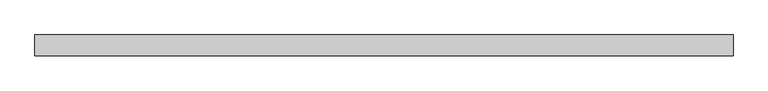
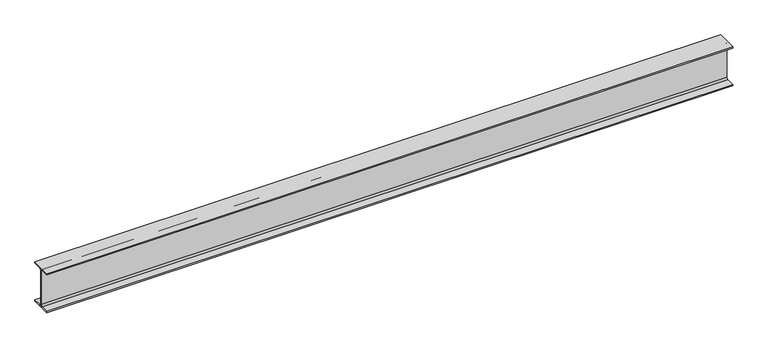
"""IFC4 building model written with IfcOpenShell, lengths in millimetres: beam geometry, 0912_Steel Framing_H-KSD3502 : H_SB_ASB_H-350x175x7x11."""

from ifc_helpers import new_model, si_unit, point, frame, frame_2d, origin, place, context, project, spatial, polyline, circle_curve, trimmed, segment, composite_curve, outline, extrude, source, transform, mapped, element, save


def beam_b532c406(model_context):
    return source(origin(), model_context, "Body", "SweptSolid", [
        extrude(outline(composite_curve([segment(polyline([(87.5, -164.0), (87.5, -175.0), (-87.5, -175.0), (-87.5, -164.0), (-17.5, -164.0)]), True, "CONTINUOUS"), segment(trimmed(circle_curve(frame_2d((-17.5, -150.0)), 14.0), [point((-17.5, -164.0))], [point((-3.5, -150.0))], True, "CARTESIAN"), True, "CONTINUOUS"), segment(polyline([(-3.5, -150.0), (-3.5, 150.0)]), True, "CONTINUOUS"), segment(trimmed(circle_curve(frame_2d((-17.5, 150.0)), 14.0), [point((-3.5, 150.0))], [point((-17.5, 164.0))], True, "CARTESIAN"), True, "CONTINUOUS"), segment(polyline([(-17.5, 164.0), (-87.5, 164.0), (-87.5, 175.0), (87.5, 175.0), (87.5, 164.0), (17.5, 164.0)]), True, "CONTINUOUS"), segment(trimmed(circle_curve(frame_2d((17.5, 150.0)), 14.0), [point((17.5, 164.0))], [point((3.5, 150.0))], True, "CARTESIAN"), True, "CONTINUOUS"), segment(polyline([(3.5, 150.0), (3.5, -150.0)]), True, "CONTINUOUS"), segment(trimmed(circle_curve(frame_2d((17.5, -150.0)), 14.0), [point((3.5, -150.0))], [point((17.5, -164.0))], True, "CARTESIAN"), True, "CONTINUOUS"), segment(polyline([(17.5, -164.0), (87.5, -164.0)]), True, "CONTINUOUS")], self_intersect=False)), frame((-2774.336211, 0.0, 0.0), z_axis=(1.0, 0.0, 0.0), x_axis=(0.0, 1.0, 0.0)), (0.0, 0.0, 1.0), 5797.2714142),
    ])


if __name__ == "__main__":
    model = new_model("IFC4")
    model_context = context("Model", 3, world=origin())
    ifc_project = project(units=[si_unit("LENGTHUNIT", "METRE", prefix="MILLI")], contexts=[model_context])
    site = spatial("IfcSite", under=ifc_project)
    building = spatial("IfcBuilding", under=site)
    placement = place(None, origin())
    beam_shape = beam_b532c406(model_context)
    element("IfcBeam", 1, ObjectType="0912_Steel Framing_H-KSD3502 : H_SB_ASB_H-350x175x7x11", at=placement, inside=building, context=model_context, shape_type="MappedRepresentation", body=[
        mapped(beam_shape, transform((0.0, 0.0, 0.0), x_axis=(1.0, 0.0, 0.0), y_axis=(0.0, 1.0, 0.0), z_axis=(0.0, 0.0, 1.0))),
    ])
    save(model, "model.ifc")

# Revit data of these elements
# Type "0912_Steel Framing_H-KSD3502 : H_SB_ASB_H-350x175x7x11"
#   H_WM Code_1 = "S01AA002-00001 | Main Steel Structure Fabrication Work | Shelter/Building | Medium Steel - Standard (90KG/M>Weight≥30KG/M) | Material: (   )"
#   H_WM Code_2 = "S03AA028-00001 | Main Steel Structure Erection Work | Shelter/Building | Medium Steel (90KG/M>Weight≥30KG/M) | Material: (   )"
#   H_WM Code_3 = "S01AA010-00001 | Main Steel Structure Fabrication Work | Shelter/Building | Steel Painting/Coating | for Non-Fireproofed Steel Surface, Surface Preparation, Primer, Second & Final Coat | Material: (   )"
#   H_Q'ty Cal Type Tag = "SB-Q2"
#   Width = 17.5 cm
#   Web Thickness = 0.7 cm
#   Web Fillet = 1.4 cm
#   Warping Constant = 282000.0 cm⁶
#   W = 0
#   Torsional Moment of Inertia = 19.4042 cm⁴
#   Section Area = 63.14 cm²
#   Plastic Modulus weak axis = 174.0 cm³
#   Plastic Modulus strong axis = 868.0 cm³
#   Perimeter = 1.36 m²/m
#   Nominal Weight = 49.60 kgf/m
#   Moment of Inertia weak axis = 984.00 cm⁴
#   Moment of Inertia strong axis = 13600.00 cm⁴
#   Height = 35.0 cm
#   Flange Thickness = 1.1 cm
#   Elastic Modulus weak axis = 112.0 cm³
#   Elastic Modulus strong axis = 775.0 cm³
#   Centroid Vertical = 17.5 cm
#   Centroid Horizontal = 8.75 cm
#   Ix = 136000000
#   Length [instance default] = 1.5240 m
#   Zx = 868000
#   b = 0.1750 m
#   h = 0.3500 m
#   r = 0.0140 m
#   s = 0.0070 m
#   t = 0.0110 m
#   A = 0.006314 m²
#   Structural Material [instance default] = Steel, 45-345
#   Assembly Code = ""
# Element 1 (IfcBeam, "0912_Steel Framing_H-KSD3502 : H_SB_ASB_H-350x175x7x11")
#   Structural Material = none
# Materials
#   "Steel, 45-345": class "Metal", colour RGB 189 187 185, transparency 0, Description = "Steel 345 MPa", Cost = 0
